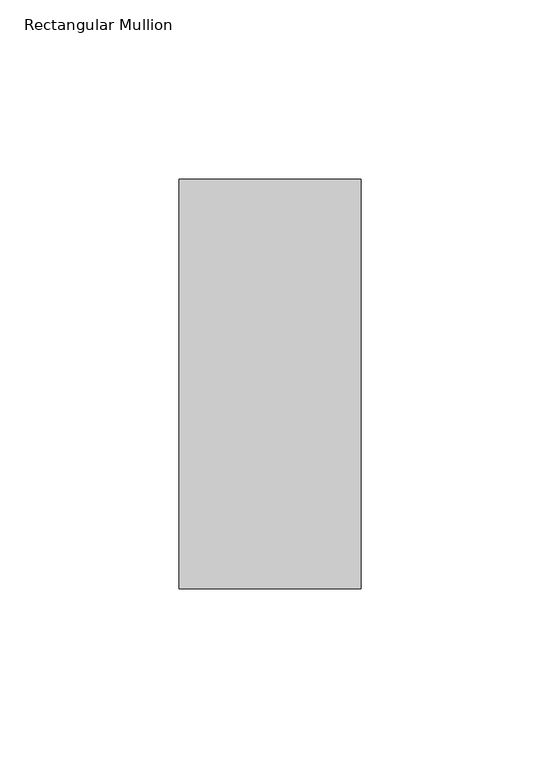
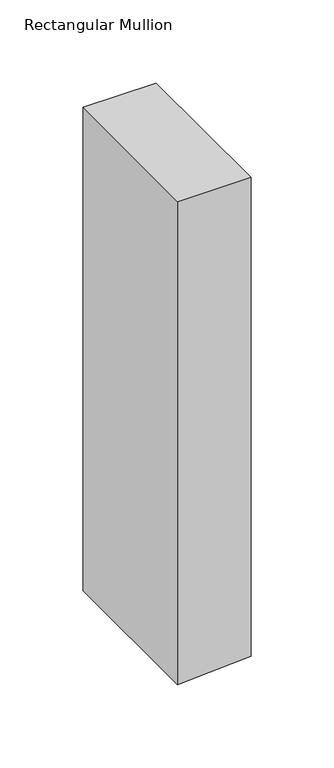
"""IFC4 building model written with IfcOpenShell, lengths in millimetres: member geometry, Rectangular Mullion : KAWNEER TRIFAB VERSAGLAZE 451T - CLEAR ANODIZED ALUM. - BACK GLAZED."""

from ifc_helpers import new_model, si_unit, frame, origin, place, context, project, spatial, polyline, outline, extrude, source, transform, mapped, element, save


def rectangular_mullion_a23bc96f(model_context):
    return source(origin(), model_context, "Body", "SweptSolid", [
        extrude(outline(polyline([(0.0, 25.4), (0.0, -25.4), (-355.3520498, -25.4), (-353.9626009, -3.1688169), (-352.1770498, 25.4), (0.0, 25.4)])), frame((0.0, -57.15, 0.0), z_axis=(0.0, 1.0, 0.0), x_axis=(0.0, 0.0, 1.0)), (0.0, 0.0, 1.0), 114.3),
    ])


if __name__ == "__main__":
    model = new_model("IFC4")
    model_context = context("Model", 3, world=origin())
    ifc_project = project(units=[si_unit("LENGTHUNIT", "METRE", prefix="MILLI")], contexts=[model_context])
    site = spatial("IfcSite", under=ifc_project)
    building = spatial("IfcBuilding", under=site)
    placement = place(None, origin())
    rectangular_mullion_shape = rectangular_mullion_a23bc96f(model_context)
    element("IfcMember", 1, ObjectType="Rectangular Mullion : KAWNEER TRIFAB VERSAGLAZE 451T - CLEAR ANODIZED ALUM. - BACK GLAZED", at=placement, inside=building, context=model_context, shape_type="MappedRepresentation", body=[
        mapped(rectangular_mullion_shape, transform((0.0, 0.0, 0.0), x_axis=(1.0, 0.0, 0.0), y_axis=(0.0, 1.0, 0.0), z_axis=(0.0, 0.0, 1.0))),
    ])
    save(model, "model.ifc")

# Revit data of these elements
# Type "Rectangular Mullion : KAWNEER TRIFAB VERSAGLAZE 451T - CLEAR ANODIZED ALUM. - BACK GLAZED"
#   built-in parameter 1007304 = 0.375 (stored number, unit not read)
#   built-in parameter 1007301 = 0.0833333 (stored number, unit not read)
#   built-in parameter 1007300 = 0.0833333 (stored number, unit not read)
# Element 1 (IfcMember, "Rectangular Mullion : KAWNEER TRIFAB VERSAGLAZE 451T - CLEAR ANODIZED ALUM. - BACK GLAZED")
#   Materials on its faces: "KAWNEER TRIFAB VERSAGLAZE 451T - CLEAR ANODIZED ALUM. - BACK GLAZED"
# Materials
#   "KAWNEER TRIFAB VERSAGLAZE 451T - CLEAR ANODIZED ALUM. - BACK GLAZED": class "Metal", colour RGB 244 244 244, transparency 0, Description = "Aluminum 6061", Cost = 0
